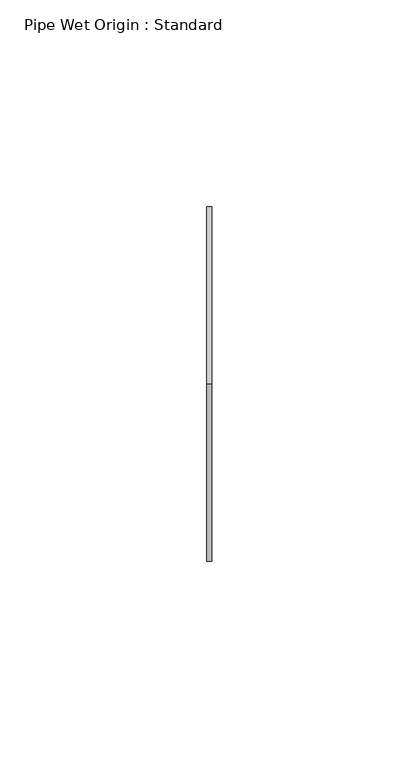
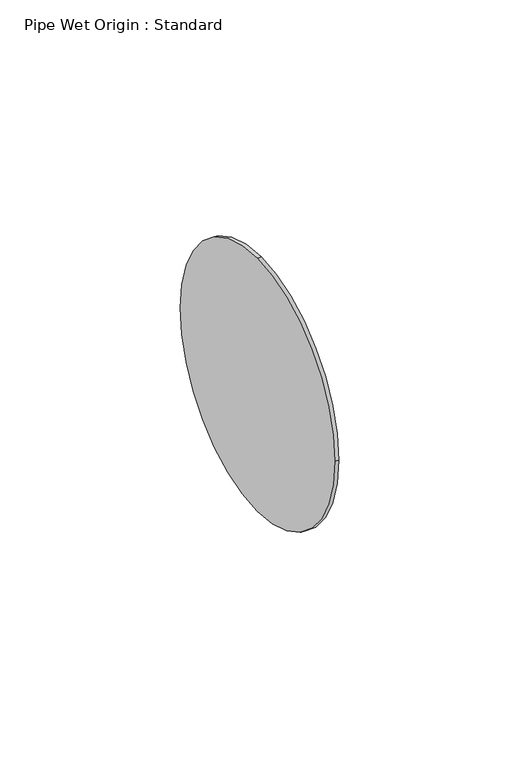
"""IFC4 building model written with IfcOpenShell, lengths in millimetres: proxy geometry, Pipe Wet Origin : Standard."""

from ifc_helpers import new_model, si_unit, point, frame, origin, origin_2d, place, context, project, spatial, circle_curve, trimmed, segment, composite_curve, outline, extrude, source, transform, mapped, element, save


def pipe_wet_origin_standard_e697f1e6(model_context):
    return source(origin(), model_context, "Body", "SweptSolid", [
        extrude(outline(composite_curve([segment(trimmed(circle_curve(origin_2d(), 42.8625), [point((0.0, 42.8625))], [point((42.8625, 0.0))], False, "CARTESIAN"), True, "CONTINUOUS"), segment(trimmed(circle_curve(origin_2d(), 42.8625), [point((42.8625, 0.0))], [point((0.0, -42.8625))], False, "CARTESIAN"), True, "CONTINUOUS"), segment(trimmed(circle_curve(origin_2d(), 42.8625), [point((0.0, -42.8625))], [point((-42.8625, 0.0))], False, "CARTESIAN"), True, "CONTINUOUS"), segment(trimmed(circle_curve(origin_2d(), 42.8625), [point((-42.8625, 0.0))], [point((0.0, 42.8625))], False, "CARTESIAN"), True, "CONTINUOUS")], self_intersect=False)), frame((0.0, 0.0, 0.0), z_axis=(1.0, 0.0, 0.0), x_axis=(0.0, 1.0, 0.0)), (0.0, 0.0, 1.0), 1.27),
        extrude(outline(composite_curve([segment(trimmed(circle_curve(origin_2d(), 42.8625), [point((0.0, 42.8625))], [point((42.8625, 0.0))], False, "CARTESIAN"), True, "CONTINUOUS"), segment(trimmed(circle_curve(origin_2d(), 42.8625), [point((42.8625, 0.0))], [point((0.0, -42.8625))], False, "CARTESIAN"), True, "CONTINUOUS"), segment(trimmed(circle_curve(origin_2d(), 42.8625), [point((0.0, -42.8625))], [point((-42.8625, 0.0))], False, "CARTESIAN"), True, "CONTINUOUS"), segment(trimmed(circle_curve(origin_2d(), 42.8625), [point((-42.8625, 0.0))], [point((0.0, 42.8625))], False, "CARTESIAN"), True, "CONTINUOUS")], self_intersect=False)), frame((0.0, 0.0, 0.0), z_axis=(1.0, 0.0, 0.0), x_axis=(0.0, 1.0, 0.0)), (0.0, 0.0, 1.0), 1.27),
    ])


if __name__ == "__main__":
    model = new_model("IFC4")
    model_context = context("Model", 3, world=origin())
    ifc_project = project(units=[si_unit("LENGTHUNIT", "METRE", prefix="MILLI")], contexts=[model_context])
    site = spatial("IfcSite", under=ifc_project)
    building = spatial("IfcBuilding", under=site)
    placement = place(None, origin())
    pipe_wet_origin_standard_shape = pipe_wet_origin_standard_e697f1e6(model_context)
    element("IfcBuildingElementProxy", 1, Name="Pipe Wet Origin : Standard", ObjectType="Pipe Wet Origin : Standard", at=placement, inside=building, context=model_context, shape_type="MappedRepresentation", body=[
        mapped(pipe_wet_origin_standard_shape, transform((0.0, 0.0, 0.0), x_axis=(1.0, 0.0, 0.0), y_axis=(0.0, 1.0, 0.0), z_axis=(0.0, 0.0, 1.0))),
    ])
    save(model, "model.ifc")

# Revit data of these elements
# Type "Pipe Wet Origin : Standard"
#   Lookup Table Name [instance default] = "Pipe Fitting Sizes"
#   WaterFlow [instance default] = 0 GPM
#   Radius [instance default] = 2 3/16"
#   Nominal Size [instance default] = 4"
#   Nominal Radius [instance default] = 2"
#   Insulation Thickness [instance default] = 0"
#   Insulation Radius [instance default] = 2 3/16"
#   IsCustom [instance default] = no
#   Assembly Code = ""
# Element 1 (IfcBuildingElementProxy, "Pipe Wet Origin : Standard")
#   Radius = 1 11/16"
#   Nominal Size = 3"
#   Nominal Radius = 1 1/2"
#   Insulation Radius = 1 11/16"
